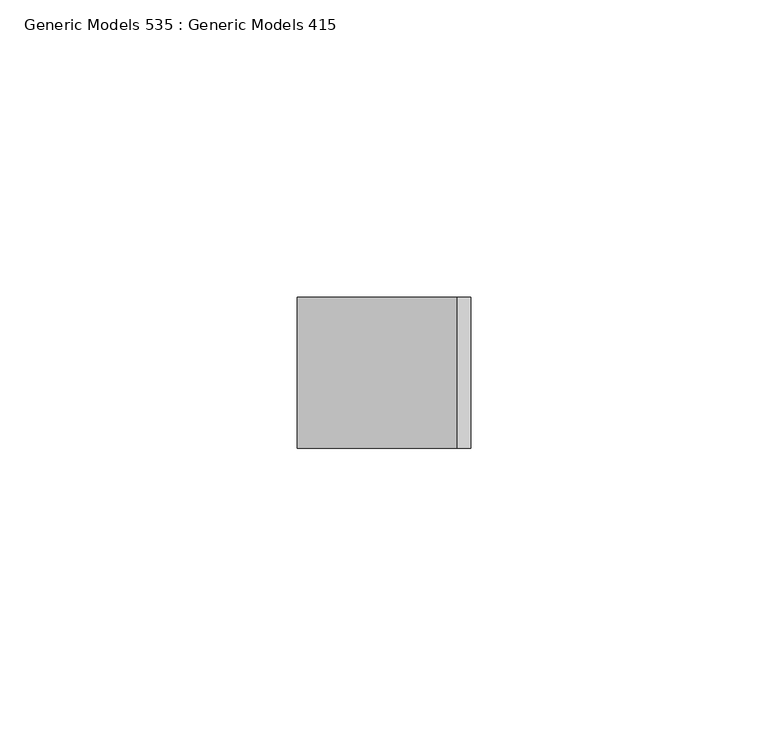
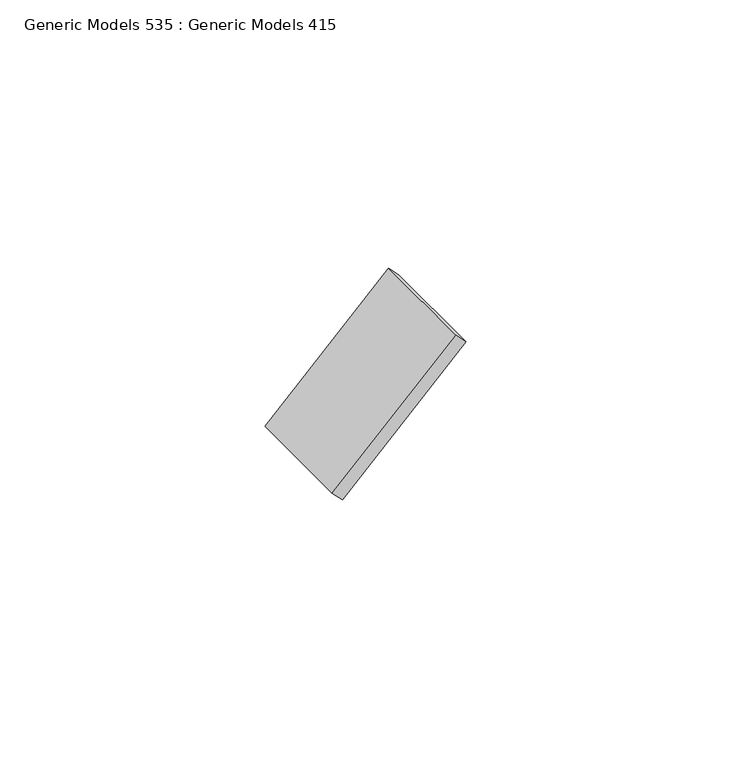
"""IFC4 building model written with IfcOpenShell, lengths in millimetres: proxy geometry, Generic Models 535 : Generic Models 415."""

from ifc_helpers import new_model, si_unit, frame, origin, place, context, project, spatial, polyline, outline, extrude, source, transform, mapped, element, save


def generic_models_535_generic_models_415_8e2e56b2(model_context):
    return source(origin(), model_context, "Body", "SweptSolid", [
        extrude(outline(polyline([(0.0, -3.175), (0.0, 0.0), (25.4, 0.0), (25.4, -3.175), (0.0, -3.175)])), frame((7848.0411784, 4501.3863946, 125194.3849742), z_axis=(0.7071067811867181, 0.0, 0.707106781186377), x_axis=(0.0, -1.0, 0.0)), (0.0, 0.0, 1.0), 38.1),
    ])


if __name__ == "__main__":
    model = new_model("IFC4")
    model_context = context("Model", 3, world=origin())
    ifc_project = project(units=[si_unit("LENGTHUNIT", "METRE", prefix="MILLI")], contexts=[model_context])
    site = spatial("IfcSite", under=ifc_project)
    building = spatial("IfcBuilding", under=site)
    placement = place(None, origin())
    generic_models_535_generic_models_415_shape = generic_models_535_generic_models_415_8e2e56b2(model_context)
    element("IfcBuildingElementProxy", 1, Name="Generic Models 535 : Generic Models 415", ObjectType="Generic Models 535 : Generic Models 415", at=placement, inside=building, context=model_context, shape_type="MappedRepresentation", body=[
        mapped(generic_models_535_generic_models_415_shape, transform((0.0, 0.0, 0.0), x_axis=(1.0, 0.0, 0.0), y_axis=(0.0, 1.0, 0.0), z_axis=(0.0, 0.0, 1.0))),
    ])
    save(model, "model.ifc")

# Revit data of these elements
# Element 1 (IfcBuildingElementProxy, "Generic Models 535 : Generic Models 415")
#   Materials on its faces: "_WELDED STEEL TABS FOR LOUVER ATTACHMENT"
# Materials
#   "_WELDED STEEL TABS FOR LOUVER ATTACHMENT": class "Metal", colour RGB 199 199 199, transparency 0, Description = "Structural steel 50ksi", Cost = 0
